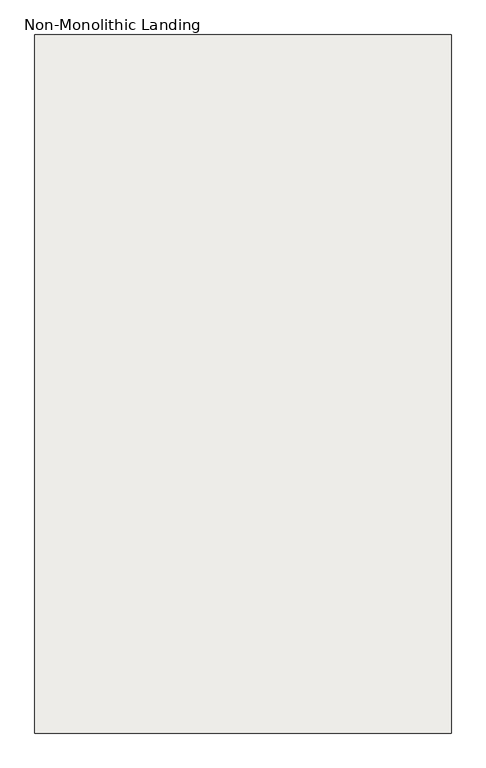
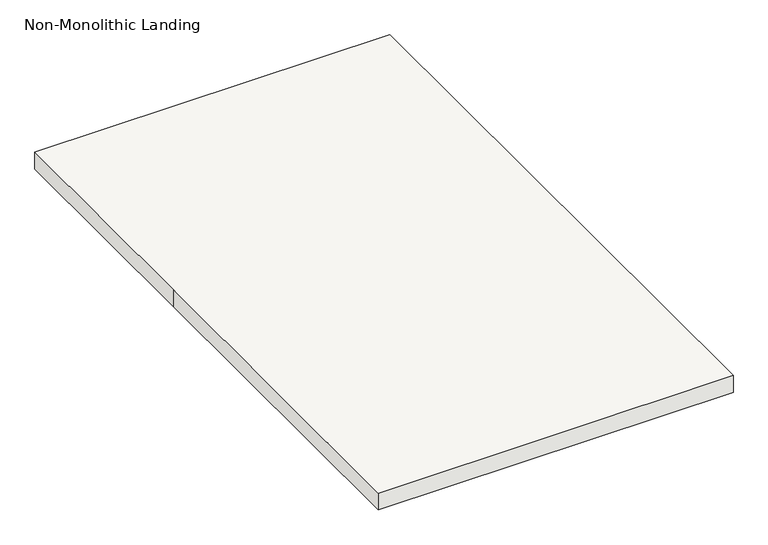
"""IFC4 building model written with IfcOpenShell, lengths in millimetres: slab geometry, Non-Monolithic Landing."""

from ifc_helpers import new_model, si_unit, frame, origin, place, context, project, spatial, polyline, outline, extrude, source, transform, mapped, element, save


def non_monolithic_landing_56f0a20b(model_context):
    return source(origin(), model_context, "Body", "SweptSolid", [
        extrude(outline(polyline([(21749.836337, -3576.2808257), (21749.836337, -2900.524372), (22749.836337, -2900.524372), (22749.836337, -4576.2808257), (21749.836337, -4576.2808257), (21749.836337, -3576.2808257)])), frame((0.0, 0.0, 1859.0909091), z_axis=(0.0, 0.0, 1.0), x_axis=(1.0, 0.0, 0.0)), (0.0, 0.0, 1.0), 50.0),
    ])


if __name__ == "__main__":
    model = new_model("IFC4")
    model_context = context("Model", 3, world=origin())
    ifc_project = project(units=[si_unit("LENGTHUNIT", "METRE", prefix="MILLI")], contexts=[model_context])
    site = spatial("IfcSite", under=ifc_project)
    building = spatial("IfcBuilding", under=site)
    placement = place(None, origin())
    non_monolithic_landing_shape = non_monolithic_landing_56f0a20b(model_context)
    element("IfcSlab", 1, ObjectType="Non-Monolithic Landing", at=placement, inside=building, context=model_context, shape_type="MappedRepresentation", body=[
        mapped(non_monolithic_landing_shape, transform((0.0, 0.0, 0.0), x_axis=(1.0, 0.0, 0.0), y_axis=(0.0, 1.0, 0.0), z_axis=(0.0, 0.0, 1.0))),
    ])
    save(model, "model.ifc")
